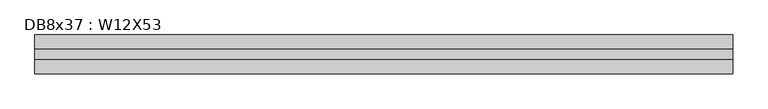
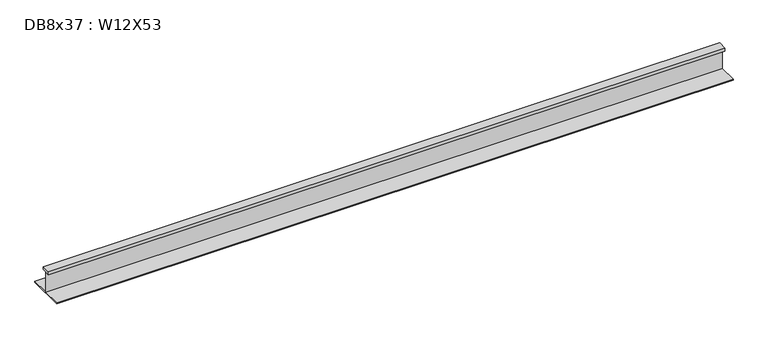
"""IFC4 building model written with IfcOpenShell, lengths in millimetres: beam geometry, DB8x37 : W12X53."""

from ifc_helpers import new_model, si_unit, frame, origin, place, context, project, spatial, polyline, outline, extrude, source, transform, mapped, element, save


def db8x37_w12x53_eecb3670(model_context):
    return source(origin(), model_context, "Body", "SweptSolid", [
        extrude(outline(polyline([(38.1, 145.415), (38.1, 120.015), (2.921, 120.015), (2.921, -48.4505), (152.4, -48.4505), (152.4, -58.1025), (-152.4, -58.1025), (-152.4, -48.4505), (-2.921, -48.4505), (-2.921, 120.015), (-38.1, 120.015), (-38.1, 145.415), (38.1, 145.415)])), frame((-2743.073, 0.0, 0.0), z_axis=(1.0, 0.0, 0.0), x_axis=(0.0, 1.0, 0.0)), (0.0, 0.0, 1.0), 5486.146),
    ])


if __name__ == "__main__":
    model = new_model("IFC4")
    model_context = context("Model", 3, world=origin())
    ifc_project = project(units=[si_unit("LENGTHUNIT", "METRE", prefix="MILLI")], contexts=[model_context])
    site = spatial("IfcSite", under=ifc_project)
    building = spatial("IfcBuilding", under=site)
    placement = place(None, origin())
    db8x37_w12x53_shape = db8x37_w12x53_eecb3670(model_context)
    element("IfcBeam", 1, ObjectType="DB8x37 : W12X53", at=placement, inside=building, context=model_context, shape_type="MappedRepresentation", body=[
        mapped(db8x37_w12x53_shape, transform((0.0, 0.0, 0.0), x_axis=(1.0, 0.0, 0.0), y_axis=(0.0, 1.0, 0.0), z_axis=(0.0, 0.0, 1.0))),
    ])
    save(model, "model.ifc")

# Revit data of these elements
# Type "DB8x37 : W12X53"
#   Assembly Code = "B10"
#   W = 53
#   Length [instance default] = 5' - 0"
#   bf = 0' - 10"
#   d = 1' - 0.1"
#   k = 0' - 1 3/8"
#   k2 = 0' - 0.8"
#   tf = 0' - 0.575"
#   tw = 0' - 0.345"
#   A = 0.108333 SF
#   Structural Material [instance default] = Steel ASTM A992
# Element 1 (IfcBeam, "DB8x37 : W12X53")
#   Materials on its faces: "Steel ASTM A992"
# Materials
#   "Steel ASTM A992": class "Metal", colour RGB 199 199 199, transparency 0, Description = "Structural steel 50ksi", Cost = 0
